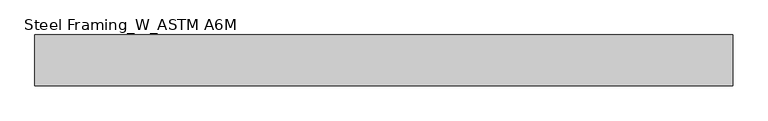
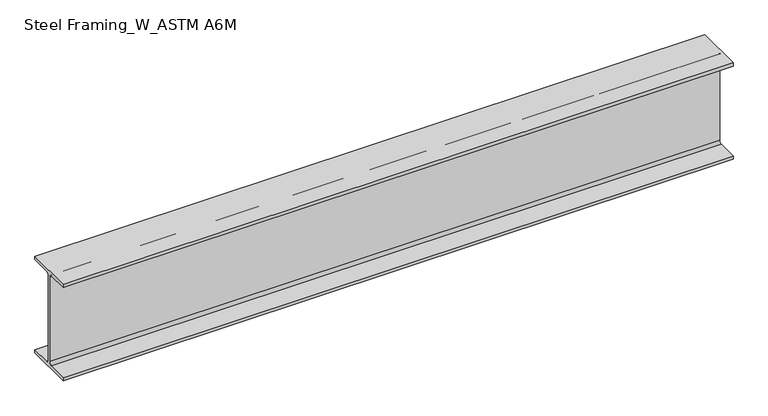
"""IFC4 building model written with IfcOpenShell, lengths in millimetres: beam geometry, Steel Framing_W_ASTM A6M : H_SB_AR_S02_W360x51_G3."""

from ifc_helpers import new_model, si_unit, point, frame, frame_2d, origin, place, context, project, spatial, polyline, circle_curve, trimmed, segment, composite_curve, outline, extrude, source, transform, mapped, element, save


def steel_framing_w_astm_a6m_761fb5d6(model_context):
    return source(origin(), model_context, "Body", "SweptSolid", [
        extrude(outline(composite_curve([segment(polyline([(85.5, -166.4), (85.5, -178.0), (-85.5, -178.0), (-85.5, -166.4), (-13.72, -166.4)]), True, "CONTINUOUS"), segment(trimmed(circle_curve(frame_2d((-13.72, -156.3)), 10.1), [point((-13.72, -166.4))], [point((-3.62, -156.3))], True, "CARTESIAN"), True, "CONTINUOUS"), segment(polyline([(-3.62, -156.3), (-3.62, 156.3)]), True, "CONTINUOUS"), segment(trimmed(circle_curve(frame_2d((-13.72, 156.3)), 10.1), [point((-3.62, 156.3))], [point((-13.72, 166.4))], True, "CARTESIAN"), True, "CONTINUOUS"), segment(polyline([(-13.72, 166.4), (-85.5, 166.4), (-85.5, 178.0), (85.5, 178.0), (85.5, 166.4), (13.72, 166.4)]), True, "CONTINUOUS"), segment(trimmed(circle_curve(frame_2d((13.72, 156.3)), 10.1), [point((13.72, 166.4))], [point((3.62, 156.3))], True, "CARTESIAN"), True, "CONTINUOUS"), segment(polyline([(3.62, 156.3), (3.62, -156.3)]), True, "CONTINUOUS"), segment(trimmed(circle_curve(frame_2d((13.72, -156.3)), 10.1), [point((3.62, -156.3))], [point((13.72, -166.4))], True, "CARTESIAN"), True, "CONTINUOUS"), segment(polyline([(13.72, -166.4), (85.5, -166.4)]), True, "CONTINUOUS")], self_intersect=False)), frame((-1003.8, 0.0, 0.0), z_axis=(1.0, 0.0, 0.0), x_axis=(0.0, 1.0, 0.0)), (0.0, 0.0, 1.0), 2339.3),
    ])


if __name__ == "__main__":
    model = new_model("IFC4")
    model_context = context("Model", 3, world=origin())
    ifc_project = project(units=[si_unit("LENGTHUNIT", "METRE", prefix="MILLI")], contexts=[model_context])
    site = spatial("IfcSite", under=ifc_project)
    building = spatial("IfcBuilding", under=site)
    placement = place(None, origin())
    steel_framing_w_astm_a6m_shape = steel_framing_w_astm_a6m_761fb5d6(model_context)
    element("IfcBeam", 1, ObjectType="Steel Framing_W_ASTM A6M : H_SB_AR_S02_W360x51_G3", at=placement, inside=building, context=model_context, shape_type="MappedRepresentation", body=[
        mapped(steel_framing_w_astm_a6m_shape, transform((0.0, 0.0, 0.0), x_axis=(1.0, 0.0, 0.0), y_axis=(0.0, 1.0, 0.0), z_axis=(0.0, 0.0, 1.0))),
    ])
    save(model, "model.ifc")

# Revit data of these elements
# Type "Steel Framing_W_ASTM A6M : H_SB_AR_S02_W360x51_G3"
#   Type Mark = "G3"
#   Section Name Key = "W14x34"
#   Width = 17.1 cm
#   Web Thickness = 0.724 cm
#   Web Fillet = 1.01 cm
#   Warping Constant = 287000.0 cm⁶
#   Torsional Moment of Inertia = 23.70 cm⁴
#   Section Area = 64.5 cm²
#   Plastic Modulus weak axis = 174.0 cm³
#   Plastic Modulus strong axis = 895.0 cm³
#   Perimeter = 1.36 m²/m
#   Nominal Weight = 51.00 kgf/m
#   Moment of Inertia weak axis = 970.00 cm⁴
#   Moment of Inertia strong axis = 14200.00 cm⁴
#   Height = 35.6 cm
#   Flange Thickness = 1.16 cm
#   Elastic Modulus weak axis = 113.0 cm³
#   Elastic Modulus strong axis = 796.0 cm³
#   Centroid Vertical = 17.8 cm
#   Centroid Horizontal = 8.55 cm
#   Length [instance default] = 1500 mm
#   Structural Material [instance default] = Steel, 45-345
#   Bolt Spacing = 0
#   Assembly Code = ""
# Element 1 (IfcBeam, "Steel Framing_W_ASTM A6M : H_SB_AR_S02_W360x51_G3")
#   Materials on its faces: "Steel, 45-345"
# Materials
#   "Steel, 45-345": class "Metal", colour RGB 189 187 185, transparency 0, Description = "Steel 345 MPa", Cost = 0
